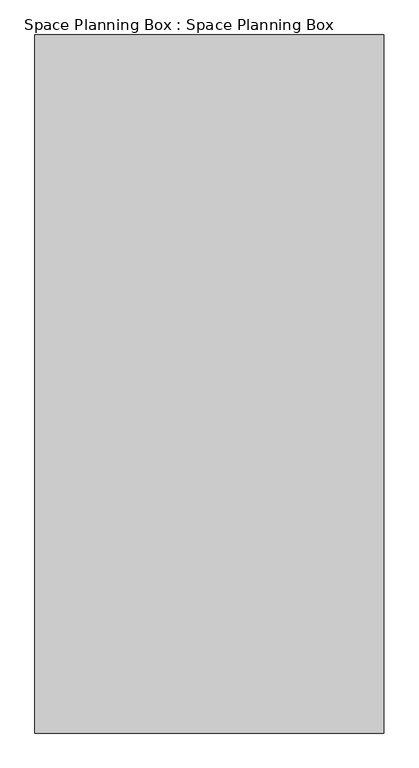
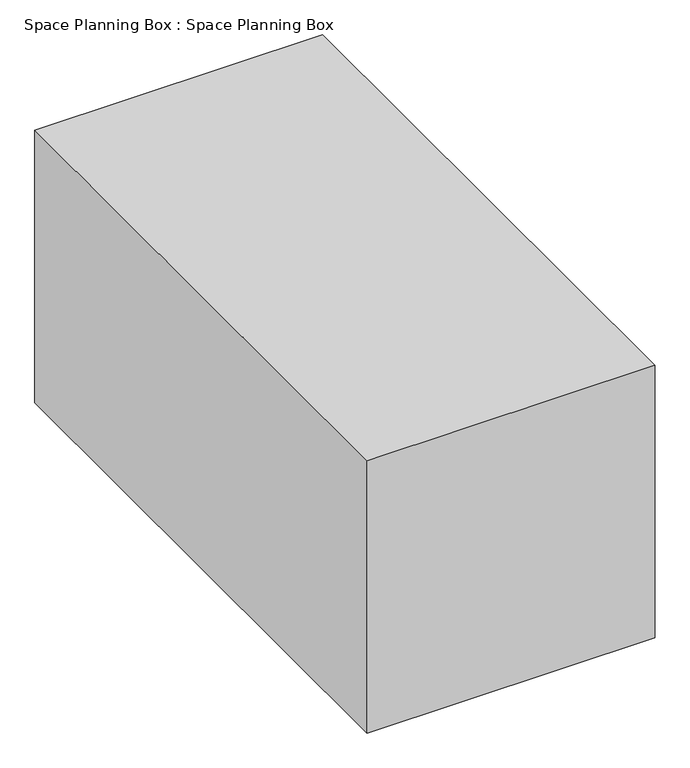
"""IFC4 building model written with IfcOpenShell, lengths in millimetres: proxy geometry, Space Planning Box : Space Planning Box."""

from ifc_helpers import new_model, si_unit, origin, origin_with_axes, place, context, project, spatial, polyline, outline, extrude, source, transform, mapped, element, save


def space_planning_box_space_planning_box_43059f4e(model_context):
    return source(origin(), model_context, "Body", "SweptSolid", [
        extrude(outline(polyline([(3000.0, 6000.0), (3000.0, -6000.0), (-3000.0, -6000.0), (-3000.0, 6000.0), (3000.0, 6000.0)])), origin_with_axes(), (0.0, 0.0, 1.0), 6000.0),
    ])


if __name__ == "__main__":
    model = new_model("IFC4")
    model_context = context("Model", 3, world=origin())
    ifc_project = project(units=[si_unit("LENGTHUNIT", "METRE", prefix="MILLI")], contexts=[model_context])
    site = spatial("IfcSite", under=ifc_project)
    building = spatial("IfcBuilding", under=site)
    placement = place(None, origin())
    space_planning_box_space_planning_box_shape = space_planning_box_space_planning_box_43059f4e(model_context)
    element("IfcBuildingElementProxy", 1, Name="Space Planning Box : Space Planning Box", ObjectType="Space Planning Box : Space Planning Box", at=placement, inside=building, context=model_context, shape_type="MappedRepresentation", body=[
        mapped(space_planning_box_space_planning_box_shape, transform((0.0, 0.0, 0.0), x_axis=(1.0, 0.0, 0.0), y_axis=(0.0, 1.0, 0.0), z_axis=(0.0, 0.0, 1.0))),
    ])
    save(model, "model.ifc")

# Revit data of these elements
# Type "Space Planning Box : Space Planning Box"
#   Type Comments = "..."
#   Room Name [instance default] = "?"
#   Assembly Code = "..."
#   Width [instance default] = 1524 mm
#   Program Area [instance default] = 0 m²
#   Length [instance default] = 1524 mm
#   Height [instance default] = 1524 mm
#   Area [instance default] = 2.32258 m²
#   Fill Color [instance default] = Cyan
#   Default Elevation = 0
# Element 1 (IfcBuildingElementProxy, "Space Planning Box : Space Planning Box")
#   Room Name = "Toilet (M)"
#   Width = 6000 mm
#   Program Area = 72 m²
#   Length = 12000 mm
#   Height = 6000 mm
#   Area = 72 m²
#   Fill Color = Lavender
#   Materials on its faces: "Lavender"
# Materials
#   "Cyan": class "Generic", colour RGB 0 255 255, transparency 0.2, Cost = 0
#   "Lavender": class "Generic", colour RGB 186 85 211, transparency 0.2, Cost = 0
